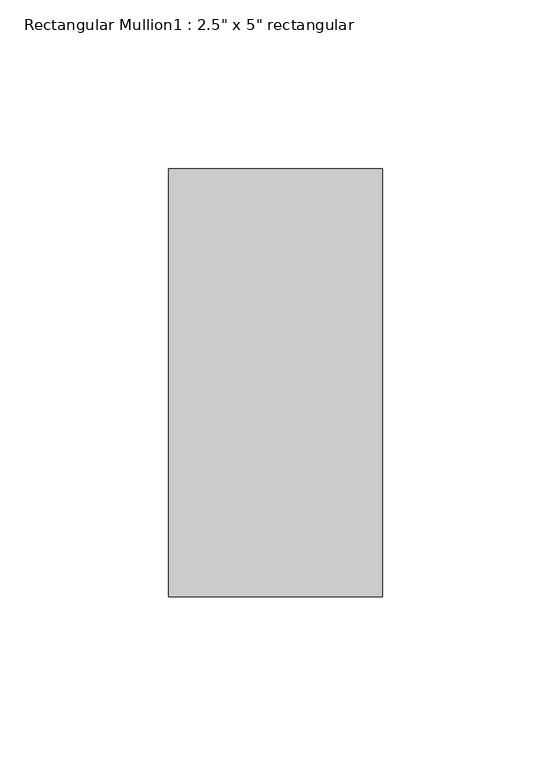
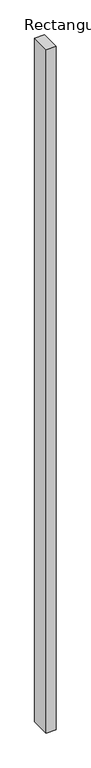
"""IFC4 building model written with IfcOpenShell, lengths in millimetres: member geometry."""

from ifc_helpers import new_model, si_unit, frame, origin, place, context, project, spatial, polyline, outline, extrude, source, transform, mapped, element, save


def member_5d07894b(model_context):
    return source(origin(), model_context, "Body", "SweptSolid", [
        extrude(outline(polyline([(31.75, 63.5), (31.75, -63.5), (-31.75, -63.5), (-31.75, 63.5), (31.75, 63.5)])), frame((0.0, 0.0, -4629.15), z_axis=(0.0, 0.0, 1.0), x_axis=(1.0, 0.0, 0.0)), (0.0, 0.0, 1.0), 4629.15),
    ])


if __name__ == "__main__":
    model = new_model("IFC4")
    model_context = context("Model", 3, world=origin())
    ifc_project = project(units=[si_unit("LENGTHUNIT", "METRE", prefix="MILLI")], contexts=[model_context])
    site = spatial("IfcSite", under=ifc_project)
    building = spatial("IfcBuilding", under=site)
    placement = place(None, origin())
    member_shape = member_5d07894b(model_context)
    element("IfcMember", 1, ObjectType="Rectangular Mullion1 : 2.5\" x 5\" rectangular", at=placement, inside=building, context=model_context, shape_type="MappedRepresentation", body=[
        mapped(member_shape, transform((0.0, 0.0, 0.0), x_axis=(1.0, 0.0, 0.0), y_axis=(0.0, 1.0, 0.0), z_axis=(0.0, 0.0, 1.0))),
    ])
    save(model, "model.ifc")

# Revit data of these elements
# Type "Rectangular Mullion1 : 2.5\" x 5\" rectangular"
#   built-in parameter 1007304 = 0.416667 (stored number, unit not read)
#   built-in parameter 1007301 = 0.104167 (stored number, unit not read)
#   built-in parameter 1007300 = 0.104167 (stored number, unit not read)
# Element 1 (IfcMember, "Rectangular Mullion1 : 2.5\" x 5\" rectangular")
#   Materials on its faces: "support-frame"
# Materials
#   "support-frame": class "Unassigned", colour RGB 233 233 233, transparency 0, Cost = 0
